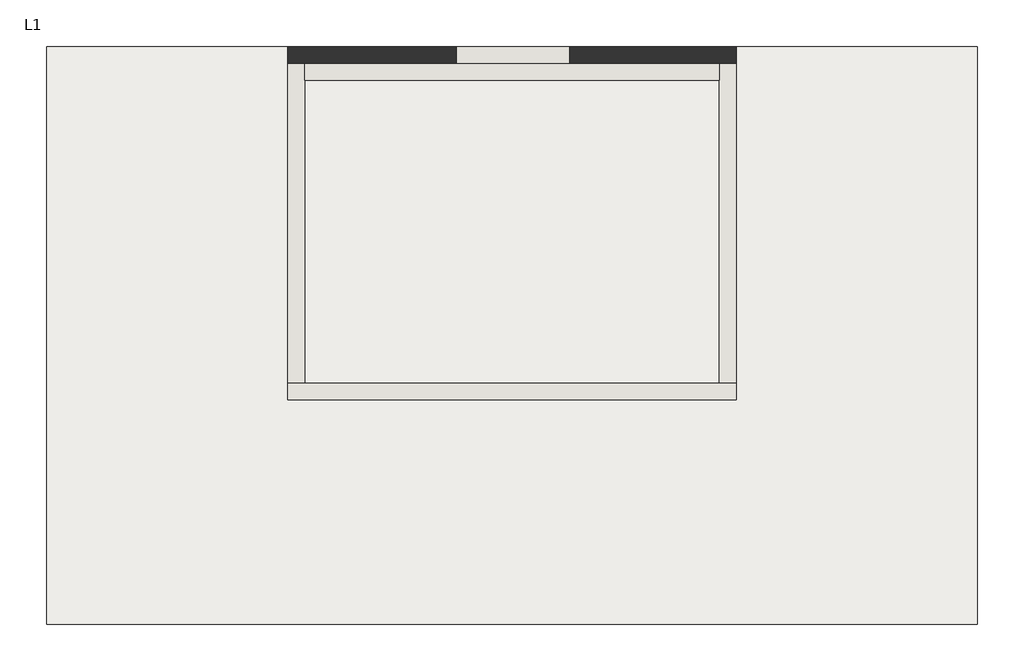
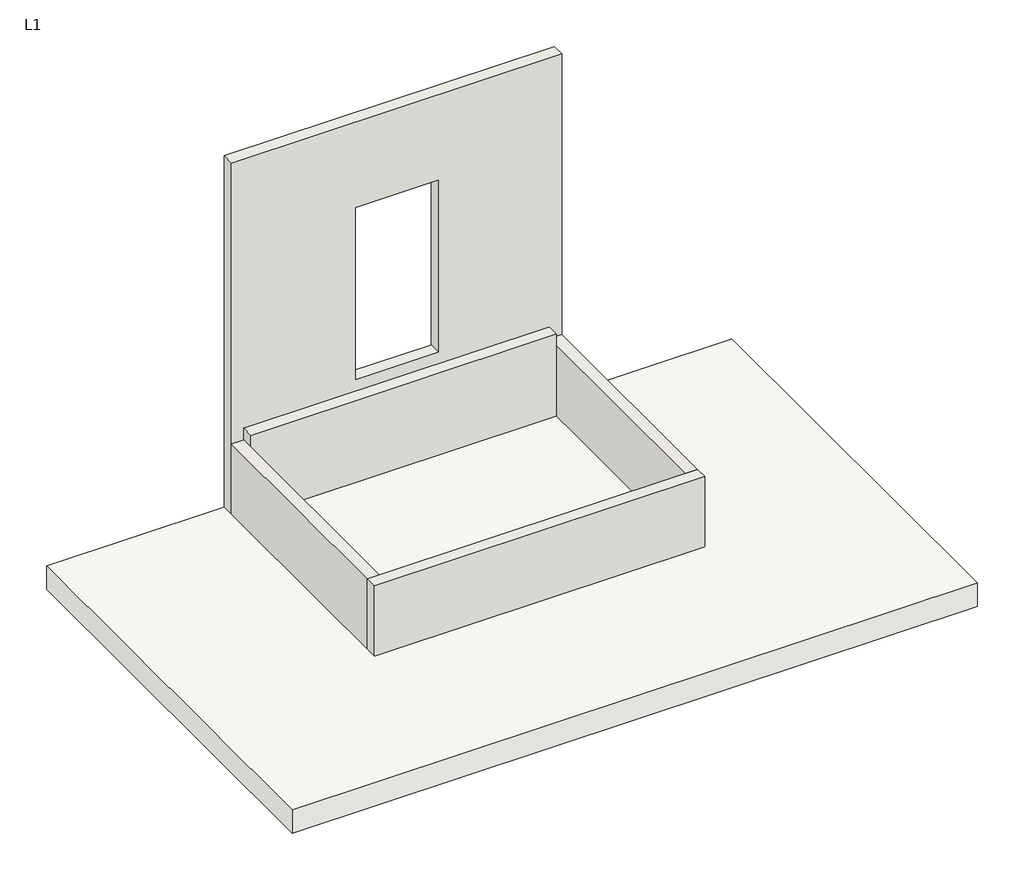
# One storey: 5 walls, 1 slab.
"""IFC4 building model written with IfcOpenShell, lengths in millimetres."""

import ifcopenshell
import ifcopenshell.guid

model = None  # the IFC model being written
_history = None  # IfcOwnerHistory: only IFC2X3 demands one
_inside = {}  # id of a spatial element -> (the spatial element, [elements in it])
_under = {}  # id of a project, library or spatial element -> (it, [spatial elements below it])
_declared = {}  # id of a project -> (the project, [libraries it declares])
_typed = {}  # id of a type object -> (the type object, [elements of that type])
_made_of = {}  # id of a material, layer set ... -> (it, [elements and type objects made of it])


def new_model(schema):
    """Start an empty IFC model of exactly this schema.

    Asked for "IFC4X3", IfcOpenShell would pick the latest addendum, in which some entities
    have other attributes; the version numbers below select the first issue.
    IFC2X3 requires an IfcOwnerHistory on every rooted entity: one is made here for all.
    """
    global model, _history
    if schema == "IFC4X3":
        model = ifcopenshell.file(schema_version=(4, 3, 0, 0))
    else:
        model = ifcopenshell.file(schema=schema)
    _inside.clear()
    _under.clear()
    _declared.clear()
    _typed.clear()
    _made_of.clear()
    _history = None
    if model.schema == "IFC2X3":
        org = make("IfcOrganization", Name="unknown")
        user = make(
            "IfcPersonAndOrganization",
            ThePerson=make("IfcPerson", FamilyName="unknown"),
            TheOrganization=org,
        )
        app = make(
            "IfcApplication",
            ApplicationDeveloper=org,
            Version="unknown",
            ApplicationFullName="unknown",
            ApplicationIdentifier="unknown",
        )
        _history = make(
            "IfcOwnerHistory",
            OwningUser=user,
            OwningApplication=app,
            ChangeAction="ADDED",
            CreationDate=0,
        )
    return model


def make(cls, **values):
    """One entity of the class cls with the attributes given. An attribute that is None is left unset."""
    return model.create_entity(
        cls, **{name: value for name, value in values.items() if value is not None}
    )


def rooted(cls, **values):
    """An entity with a GlobalId (a new one), such as an element, a storey or a relation."""
    return make(cls, GlobalId=ifcopenshell.guid.new(), OwnerHistory=_history, **values)


def si_unit(unit_type, name, prefix=None):
    """IfcSIUnit, for example si_unit("LENGTHUNIT", "METRE", prefix="MILLI")."""
    return make("IfcSIUnit", UnitType=unit_type, Prefix=prefix, Name=name)


def assignment(units):
    """IfcUnitAssignment: the units of a project."""
    return None if units is None else make("IfcUnitAssignment", Units=units)


def point(xyz):
    """IfcCartesianPoint."""
    return None if xyz is None else make("IfcCartesianPoint", Coordinates=xyz)


def direction(xyz):
    """IfcDirection."""
    return None if xyz is None else make("IfcDirection", DirectionRatios=xyz)


def frame(location, z_axis=None, x_axis=None):
    """IfcAxis2Placement3D, a coordinate frame: its origin and axes. An axis left out is left unset."""
    return make(
        "IfcAxis2Placement3D",
        Location=point(location),
        Axis=direction(z_axis),
        RefDirection=direction(x_axis),
    )


def origin():
    """The frame at (0, 0, 0) with its axes left unset."""
    return frame((0.0, 0.0, 0.0))


def place(relative_to, where):
    """IfcLocalPlacement: puts the frame where relative to a parent placement (None: the world)."""
    return make(
        "IfcLocalPlacement", PlacementRelTo=relative_to, RelativePlacement=where
    )


def context(
    kind, dimensions, precision=None, world=None, true_north=None, identifier=None
):
    """IfcGeometricRepresentationContext, for example the 3D "Model" context."""
    return make(
        "IfcGeometricRepresentationContext",
        ContextIdentifier=identifier,
        ContextType=kind,
        CoordinateSpaceDimension=dimensions,
        Precision=precision,
        WorldCoordinateSystem=world,
        TrueNorth=true_north,
    )


def project(units=None, contexts=None):
    """IfcProject with its units and contexts."""
    return rooted(
        "IfcProject",
        Name="project",
        RepresentationContexts=contexts,
        UnitsInContext=assignment(units),
    )


def spatial(cls, under=None, at=None, **own):
    """A site, building, storey or space (cls), placed at a placement, below another one or the project."""
    s = rooted(cls, ObjectPlacement=at, **own)
    if under is not None:
        _under.setdefault(under.id(), (under, []))[1].append(s)
    return s


def polyline(points):
    """IfcPolyline through the points."""
    return make("IfcPolyline", Points=[point(p) for p in points])


def outline(outer, holes=None, kind="AREA"):
    """IfcArbitraryClosedProfileDef: a profile drawn as a closed curve; with holes, ...WithVoids."""
    if holes is None:
        return make("IfcArbitraryClosedProfileDef", ProfileType=kind, OuterCurve=outer)
    return make(
        "IfcArbitraryProfileDefWithVoids",
        ProfileType=kind,
        OuterCurve=outer,
        InnerCurves=holes,
    )


def extrude(swept, where, along, depth):
    """IfcExtrudedAreaSolid: the profile swept, set in the frame where, extruded along a direction by depth."""
    return make(
        "IfcExtrudedAreaSolid",
        SweptArea=swept,
        Position=where,
        ExtrudedDirection=direction(along),
        Depth=depth,
    )


def faces_of(points, faces, orient=None, outer=None):
    """IfcFace entities. A face is a list of loops; a loop is a list of indices into points, from 0.

    orient and outer hold one flag for each loop. By default every Orientation is true, the
    first loop of a face is its IfcFaceOuterBound and the others are IfcFaceBound.
    """
    made = []
    for i, loops in enumerate(faces):
        bounds = []
        for j, loop in enumerate(loops):
            is_outer = j == 0 if outer is None else outer[i][j]
            bounds.append(
                make(
                    "IfcFaceOuterBound" if is_outer else "IfcFaceBound",
                    Bound=make("IfcPolyLoop", Polygon=[points[k] for k in loop]),
                    Orientation=True if orient is None else orient[i][j],
                )
            )
        made.append(make("IfcFace", Bounds=bounds))
    return made


def faceted_brep(points, faces, orient=None, outer=None, voids=None):
    """IfcFacetedBrep: a solid bounded by flat faces; with voids (closed shells), ...WithVoids."""
    shared = [point(p) for p in points]
    hull = make("IfcClosedShell", CfsFaces=faces_of(shared, faces, orient, outer))
    if voids is None:
        return make("IfcFacetedBrep", Outer=hull)
    return make(
        "IfcFacetedBrepWithVoids",
        Outer=hull,
        Voids=[
            make(cls, CfsFaces=faces_of(shared, fs, o, b)) for cls, fs, o, b in voids
        ],
    )


def shape(context_of_items, identifier, shape_type, items):
    """IfcShapeRepresentation: the items that make up one representation, for example the "Body"."""
    return make(
        "IfcShapeRepresentation",
        ContextOfItems=context_of_items,
        RepresentationIdentifier=identifier,
        RepresentationType=shape_type,
        Items=items,
    )


def made_of(thing, what):
    """Note that an element or type object is made of a material, layer set ...; save() writes the relation."""
    if what is not None:
        _made_of.setdefault(what.id(), (what, []))[1].append(thing)
    return thing


def element(
    cls,
    number,
    at=None,
    inside=None,
    cuts=None,
    type_object=None,
    material=None,
    context=None,
    identifier="Body",
    shape_type=None,
    held_by="IfcProductDefinitionShape",
    body=None,
    shapes=None,
    **own,
):
    """One element of the class cls, such as IfcWall. Its Tag is "e" and its number.

    at: its placement. inside: the storey or other place that contains it. cuts: it is an
    opening in that element (IfcRelVoidsElement). A single representation is given by context,
    identifier, shape_type and body (its items); several are given by shapes. held_by: the class
    of the entity that holds the representations. save() writes the other relations.
    """
    e = rooted(cls, Tag="e%d" % number, ObjectPlacement=at, **own)
    if body is not None:
        shapes = [shape(context, identifier, shape_type, body)]
    if shapes is not None:
        e.Representation = make(held_by, Representations=shapes)
    if inside is not None:
        _inside.setdefault(inside.id(), (inside, []))[1].append(e)
    if cuts is not None:
        rooted(
            "IfcRelVoidsElement", RelatingBuildingElement=cuts, RelatedOpeningElement=e
        )
    if type_object is not None:
        _typed.setdefault(type_object.id(), (type_object, []))[1].append(e)
    return made_of(e, material)


def aggregate(whole, parts):
    """IfcRelAggregates: a whole, such as a stair, and the parts it consists of."""
    return rooted("IfcRelAggregates", RelatingObject=whole, RelatedObjects=parts)


def save(model, path):
    """Write the relations noted so far, then the file.

    IfcRelAggregates (storeys below a building ...), IfcRelContainedInSpatialStructure (elements
    in a storey), IfcRelDefinesByType, IfcRelAssociatesMaterial and IfcRelDeclares: one each for
    every whole, place, type object, material and project.
    """
    for whole, parts in _under.values():
        aggregate(whole, parts)
    for where, things in _inside.values():
        rooted(
            "IfcRelContainedInSpatialStructure",
            RelatedElements=things,
            RelatingStructure=where,
        )
    for kind, things in _typed.values():
        rooted("IfcRelDefinesByType", RelatedObjects=things, RelatingType=kind)
    for what, things in _made_of.values():
        rooted("IfcRelAssociatesMaterial", RelatedObjects=things, RelatingMaterial=what)
    for by, libraries in _declared.values():
        rooted("IfcRelDeclares", RelatingContext=by, RelatedDefinitions=libraries)
    model.write(path)


model = new_model("IFC4")

# Units and contexts
model_context = context("Model", 3, world=origin())
ifc_project = project(units=[si_unit("LENGTHUNIT", "METRE", prefix="MILLI")], contexts=[model_context])

# Site, building, storey
site = spatial("IfcSite", under=ifc_project)
building = spatial("IfcBuilding", under=site)
storey = spatial("IfcBuildingStorey", under=building, Name="L1", Elevation=0.0)

# Slab
placement = place(None, origin())
element("IfcSlab", 1, ObjectType="Generic 300mm", at=placement, inside=storey, context=model_context, shape_type="SweptSolid", body=[
    extrude(outline(polyline([(4893.2318, -2858.4292912), (-3406.7682, -2858.4292912), (-3406.7682, 2291.5707088), (4893.2318, 2291.5707088), (4893.2318, -2858.4292912)])), frame((0.0, 0.0, -300.0), z_axis=(0.0, 0.0, 1.0), x_axis=(1.0, 0.0, 0.0)), (0.0, 0.0, 1.0), 300.0),
])

# Walls
element("IfcWall", 2, ObjectType="Generic - 150mm", at=placement, inside=storey, context=model_context, shape_type="Brep", body=[
    faceted_brep([(-1256.7682, -858.4292912, 0.0), (2743.2318, -858.4292912, 0.0), (2743.2318, -858.4292912, 900.0), (-1256.7682, -858.4292912, 900.0), (-1256.7682, -708.4292912, 0.0), (-1256.7682, -708.4292912, 900.0), (-1106.7682, -708.4292912, 900.0), (2593.2318, -708.4292912, 900.0), (2743.2318, -708.4292912, 900.0), (2743.2318, -708.4292912, 0.0), (2593.2318, -708.4292912, 0.0), (-1106.7682, -708.4292912, 0.0)], [[[0, 1, 2, 3]], [[4, 5, 6, 7, 8, 9, 10, 11]], [[1, 0, 4, 11, 10, 9]], [[0, 3, 5, 4]], [[2, 1, 9, 8]], [[3, 2, 8, 7, 6, 5]]]),
])
element("IfcWall", 3, ObjectType="Generic - 150mm", at=placement, inside=storey, context=model_context, shape_type="Brep", body=[
    faceted_brep([(-1106.7682, -708.4292912, 0.0), (-1106.7682, 1991.5707088, 0.0), (-1106.7682, 2141.5707088, 0.0), (-1106.7682, 2141.5707088, 900.0), (-1106.7682, -708.4292912, 900.0), (-1256.7682, -708.4292912, 0.0), (-1256.7682, -708.4292912, 900.0), (-1256.7682, 2141.5707088, 900.0), (-1256.7682, 2141.5707088, 0.0)], [[[0, 1, 2, 3, 4]], [[5, 6, 7, 8]], [[2, 1, 0, 5, 8]], [[4, 3, 7, 6]], [[0, 4, 6, 5]], [[3, 2, 8, 7]]]),
])
element("IfcWall", 4, ObjectType="Generic - 150mm", at=placement, inside=storey, context=model_context, shape_type="Brep", body=[
    faceted_brep([(2743.2318, -708.4292912, 0.0), (2743.2318, 2141.5707088, 0.0), (2743.2318, 2141.5707088, 900.0), (2743.2318, -708.4292912, 900.0), (2593.2318, -708.4292912, 0.0), (2593.2318, -708.4292912, 900.0), (2593.2318, 2141.5707088, 900.0), (2593.2318, 2141.5707088, 0.0), (2593.2318, 1991.5707088, 0.0)], [[[0, 1, 2, 3]], [[4, 5, 6, 7, 8]], [[1, 0, 4, 8, 7]], [[3, 2, 6, 5]], [[0, 3, 5, 4]], [[2, 1, 7, 6]]]),
])
element("IfcWall", 5, ObjectType="Generic - 150mm", at=placement, inside=storey, context=model_context, shape_type="Brep", body=[
    faceted_brep([(-1106.7682, 1991.5707088, 0.0), (2593.2318, 1991.5707088, 0.0), (2593.2318, 1991.5707088, 1050.0), (-1106.7682, 1991.5707088, 1050.0), (-1106.7682, 2141.5707088, 0.0), (-1106.7682, 2141.5707088, 900.0), (-1106.7682, 2141.5707088, 1050.0), (2593.2318, 2141.5707088, 1050.0), (2593.2318, 2141.5707088, 900.0), (2593.2318, 2141.5707088, 0.0)], [[[0, 1, 2, 3]], [[4, 5, 6, 7, 8, 9]], [[1, 0, 4, 9]], [[3, 2, 7, 6]], [[0, 3, 6, 5, 4]], [[2, 1, 9, 8, 7]]]),
])
element("IfcWall", 6, ObjectType="Generic - 150mm", at=placement, inside=storey, context=model_context, shape_type="Brep", body=[
    faceted_brep([(-1256.7682, 2141.5707088, 0.0), (2743.2318, 2141.5707088, 0.0), (2743.2318, 2141.5707088, 1200.0), (2743.2318, 2141.5707088, 2300.0), (2743.2318, 2141.5707088, 4500.0), (-1256.7682, 2141.5707088, 4500.0), (-1256.7682, 2141.5707088, 2300.0), (-1256.7682, 2141.5707088, 1200.0), (252.7568, 2141.5707088, 1200.0), (252.7568, 2141.5707088, 3400.0), (1252.7568, 2141.5707088, 3400.0), (1252.7568, 2141.5707088, 1200.0), (-1256.7682, 2291.5707088, 0.0), (-1256.7682, 2291.5707088, 4500.0), (2743.2318, 2291.5707088, 4500.0), (2743.2318, 2291.5707088, 0.0), (252.7568, 2291.5707088, 1200.0), (1252.7568, 2291.5707088, 1200.0), (1252.7568, 2291.5707088, 3400.0), (252.7568, 2291.5707088, 3400.0)], [[[0, 1, 2, 3, 4, 5, 6, 7], [8, 9, 10, 11]], [[12, 13, 14, 15], [16, 17, 18, 19]], [[1, 0, 12, 15]], [[5, 4, 14, 13]], [[9, 8, 16, 19]], [[10, 9, 19, 18]], [[11, 10, 18, 17]], [[8, 11, 17, 16]], [[0, 7, 6, 5, 13, 12]], [[4, 3, 2, 1, 15, 14]]]),
])

save(model, "model.ifc")

# Revit data of these elements
# Project information
#   Название организации = "Organization Name"
#   Описание организации = "Organization Description"
#   Наименование здания = "Building Name"
#   Дата утверждения проекта = "Issue Date"
#   Статус проекта = "Project Status"
#   Заказчик = "Client Name"
#   Адрес проекта = "Enter address here\nAddress Line 2"
#   Наименование проекта = "Project Name"
#   Номер проекта = "Project Number"
# Type "Generic 300mm"
#   Description = "Generic Floor (Material By Category), 300mm thick"
#   Function = 0
#   Layers, outside or top first: 300 mm no material (function 1)
# Type "Generic - 150mm"
#   Description = "Generic Wall (Material By Category), 150mm thick"
#   Type Mark = "G04"
#   Layers, outside or top first: 150 mm no material (function 1)
# Element 1 (IfcSlab, "Generic 300mm")
#   Height Offset From Level = 0 mm
#   Phase Created = New Construction
#   Materials on its faces: "Default Floor"
# Element 2 (IfcWall, "Generic - 150mm")
#   Top Offset = 0 mm
#   Base Offset = 0 mm
#   wall height = 1200 mm
#   Phase Created = New Construction
#   Base Constraint = L1
#   Top Constraint = L2
#   Materials on its faces: "Default Wall"
# Elements 3, 4 (IfcWall, "Generic - 150mm")
#   Top Offset = 0 mm
#   Base Offset = 0 mm
#   Unconnected Height = 900 mm
#   wall height = 900 mm
#   Phase Created = New Construction
#   Base Constraint = L1
#   Materials on its faces: "Default Wall"
# Element 5 (IfcWall, "Generic - 150mm")
#   Top Offset = 0 mm
#   Base Offset = 0 mm
#   Unconnected Height = 1050 mm
#   wall height = 1050 mm
#   Phase Created = New Construction
#   Base Constraint = L1
#   Materials on its faces: "Default Wall"
# Element 6 (IfcWall, "Generic - 150mm")
#   Top Offset = 0 mm
#   Base Offset = 0 mm
#   Unconnected Height = 4500 mm
#   wall height = 4500 mm
#   Phase Created = New Construction
#   Base Constraint = L1
#   Materials on its faces: "Default Wall"
# Materials
#   "Default Floor": class "Miscellaneous", colour RGB 128 128 128, transparency 0, Cost = 0
#   "Default Wall": class "Miscellaneous", colour RGB 192 192 192, transparency 0, Cost = 0
